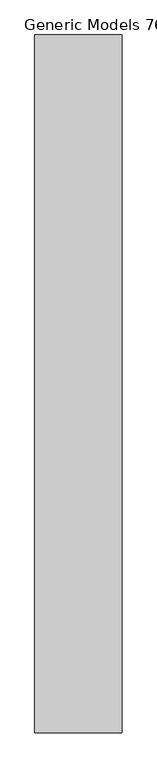
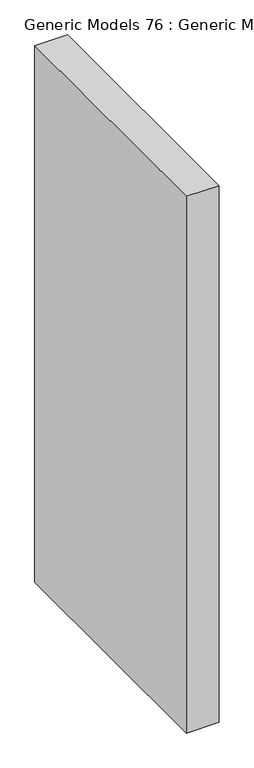
"""IFC4 building model written with IfcOpenShell, lengths in millimetres: proxy geometry, Generic Models 76 : Generic Models 1."""

from ifc_helpers import new_model, si_unit, frame, origin, place, context, project, spatial, polyline, outline, extrude, source, transform, mapped, element, save


def generic_models_76_generic_models_1_e0c76cb0(model_context):
    return source(origin(), model_context, "Body", "SweptSolid", [
        extrude(outline(polyline([(51930.3, 1219.2), (51930.3, 0.0), (51777.9, 0.0), (51777.9, 1219.2), (51930.3, 1219.2)])), frame((0.0, 0.0, 3048.0), z_axis=(0.0, 0.0, 1.0), x_axis=(1.0, 0.0, 0.0)), (0.0, 0.0, 1.0), 2633.9569015),
    ])


if __name__ == "__main__":
    model = new_model("IFC4")
    model_context = context("Model", 3, world=origin())
    ifc_project = project(units=[si_unit("LENGTHUNIT", "METRE", prefix="MILLI")], contexts=[model_context])
    site = spatial("IfcSite", under=ifc_project)
    building = spatial("IfcBuilding", under=site)
    placement = place(None, origin())
    generic_models_76_generic_models_1_shape = generic_models_76_generic_models_1_e0c76cb0(model_context)
    element("IfcBuildingElementProxy", 1, Name="Generic Models 76 : Generic Models 1", ObjectType="Generic Models 76 : Generic Models 1", at=placement, inside=building, context=model_context, shape_type="MappedRepresentation", body=[
        mapped(generic_models_76_generic_models_1_shape, transform((0.0, 0.0, 0.0), x_axis=(1.0, 0.0, 0.0), y_axis=(0.0, 1.0, 0.0), z_axis=(0.0, 0.0, 1.0))),
    ])
    save(model, "model.ifc")

# Revit data of these elements
# Element 1 (IfcBuildingElementProxy, "Generic Models 76 : Generic Models 1")
#   Materials on its faces: "CMU (SEE 'WALL TAGE' FOR SIZE)"
# Materials
#   "CMU (SEE 'WALL TAGE' FOR SIZE)": class "Masonry", colour RGB 203 203 199, transparency 0, Description = "Concrete masonry units", Cost = 0
